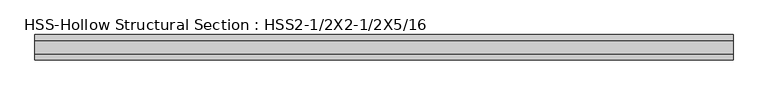
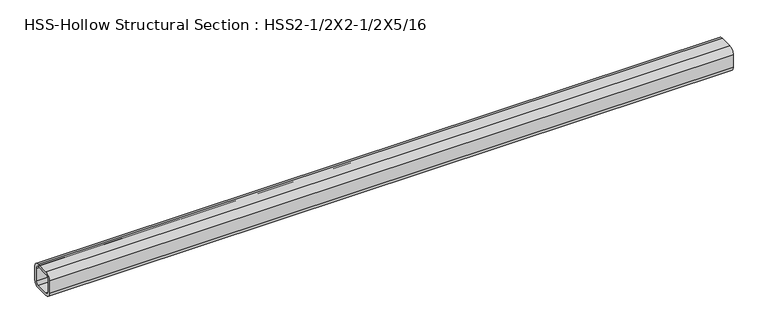
"""IFC4 building model written with IfcOpenShell, lengths in millimetres: beam geometry, HSS-Hollow Structural Section : HSS2-1/2X2-1/2X5/16."""

from ifc_helpers import new_model, si_unit, point, frame, frame_2d, origin, place, context, project, spatial, polyline, circle_curve, trimmed, segment, composite_curve, outline, extrude, source, transform, mapped, element, save


def hss_hollow_structural_section_hss2_1_2x2_1_2x5_16_5e575396(model_context):
    return source(origin(), model_context, "Body", "SweptSolid", [
        extrude(outline(composite_curve([segment(polyline([(31.75, 16.9672), (31.75, -16.9672)]), True, "CONTINUOUS"), segment(trimmed(circle_curve(frame_2d((16.9672, -16.9672)), 14.7828), [point((31.75, -16.9672))], [point((16.9672, -31.75))], False, "CARTESIAN"), True, "CONTINUOUS"), segment(polyline([(16.9672, -31.75), (-16.9672, -31.75)]), True, "CONTINUOUS"), segment(trimmed(circle_curve(frame_2d((-16.9672, -16.9672)), 14.7828), [point((-16.9672, -31.75))], [point((-31.75, -16.9672))], False, "CARTESIAN"), True, "CONTINUOUS"), segment(polyline([(-31.75, -16.9672), (-31.75, 16.9672)]), True, "CONTINUOUS"), segment(trimmed(circle_curve(frame_2d((-16.9672, 16.9672)), 14.7828), [point((-31.75, 16.9672))], [point((-16.9672, 31.75))], False, "CARTESIAN"), True, "CONTINUOUS"), segment(polyline([(-16.9672, 31.75), (16.9672, 31.75)]), True, "CONTINUOUS"), segment(trimmed(circle_curve(frame_2d((16.9672, 16.9672)), 14.7828), [point((16.9672, 31.75))], [point((31.75, 16.9672))], False, "CARTESIAN"), True, "CONTINUOUS")], self_intersect=False), holes=[composite_curve([segment(trimmed(circle_curve(frame_2d((-16.9672, 16.9672)), 7.3914), [point((-16.9672, 24.3586))], [point((-24.3586, 16.9672))], True, "CARTESIAN"), True, "CONTINUOUS"), segment(polyline([(-24.3586, 16.9672), (-24.3586, -16.9672)]), True, "CONTINUOUS"), segment(trimmed(circle_curve(frame_2d((-16.9672, -16.9672)), 7.3914), [point((-24.3586, -16.9672))], [point((-16.9672, -24.3586))], True, "CARTESIAN"), True, "CONTINUOUS"), segment(polyline([(-16.9672, -24.3586), (16.9672, -24.3586)]), True, "CONTINUOUS"), segment(trimmed(circle_curve(frame_2d((16.9672, -16.9672)), 7.3914), [point((16.9672, -24.3586))], [point((24.3586, -16.9672))], True, "CARTESIAN"), True, "CONTINUOUS"), segment(polyline([(24.3586, -16.9672), (24.3586, 16.9672)]), True, "CONTINUOUS"), segment(trimmed(circle_curve(frame_2d((16.9672, 16.9672)), 7.3914), [point((24.3586, 16.9672))], [point((16.9672, 24.3586))], True, "CARTESIAN"), True, "CONTINUOUS"), segment(polyline([(16.9672, 24.3586), (-16.9672, 24.3586)]), True, "CONTINUOUS")], self_intersect=False)]), frame((-899.0650708, 0.0, 0.0), z_axis=(1.0, 0.0, 0.0), x_axis=(0.0, 1.0, 0.0)), (0.0, 0.0, 1.0), 1741.6810272),
    ])


if __name__ == "__main__":
    model = new_model("IFC4")
    model_context = context("Model", 3, world=origin())
    ifc_project = project(units=[si_unit("LENGTHUNIT", "METRE", prefix="MILLI")], contexts=[model_context])
    site = spatial("IfcSite", under=ifc_project)
    building = spatial("IfcBuilding", under=site)
    placement = place(None, origin())
    hss_hollow_structural_section_hss2_1_2x2_1_2x5_16_shape = hss_hollow_structural_section_hss2_1_2x2_1_2x5_16_5e575396(model_context)
    element("IfcBeam", 1, ObjectType="HSS-Hollow Structural Section : HSS2-1/2X2-1/2X5/16", at=placement, inside=building, context=model_context, shape_type="MappedRepresentation", body=[
        mapped(hss_hollow_structural_section_hss2_1_2x2_1_2x5_16_shape, transform((0.0, 0.0, 0.0), x_axis=(1.0, 0.0, 0.0), y_axis=(0.0, 1.0, 0.0), z_axis=(0.0, 0.0, 1.0))),
    ])
    save(model, "model.ifc")

# Revit data of these elements
# Type "HSS-Hollow Structural Section : HSS2-1/2X2-1/2X5/16"
#   Assembly Code = "B10"
#   Shape = "Square"
#   W = 8.4
#   Ht = 0' - 2 1/2"
#   Length [instance default] = 5' - 0"
#   b = 0' - 2 1/2"
#   kr = 0' - 0.582"
#   t = 0' - 0.291"
#   A = 0.0163194 SF
#   Structural Material [instance default] = Steel ASTM A500, Grade B, Rectangular and Square
# Element 1 (IfcBeam, "HSS-Hollow Structural Section : HSS2-1/2X2-1/2X5/16")
#   Materials on its faces: "Steel ASTM A500, Grade B, Rectangular and Square"
# Materials
#   "Steel ASTM A500, Grade B, Rectangular and Square": class "Metal", colour RGB 199 199 199, transparency 0, Description = "Carbon steel", Cost = 0
